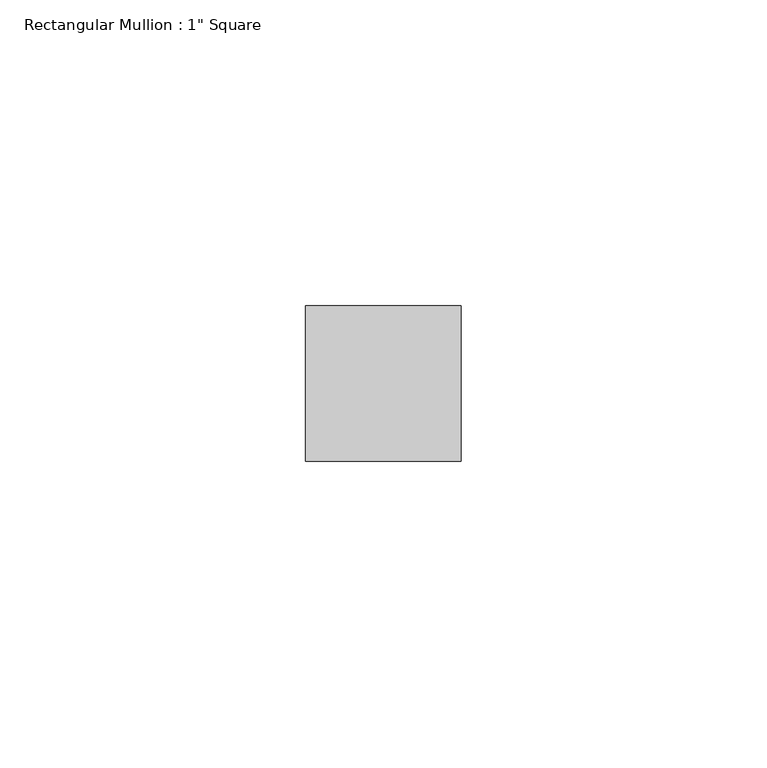
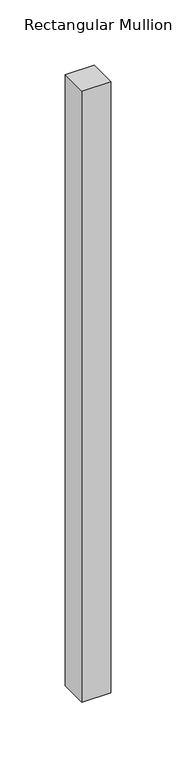
"""IFC4 building model written with IfcOpenShell, lengths in millimetres: member geometry."""

from ifc_helpers import new_model, si_unit, frame, origin, place, context, project, spatial, polyline, outline, extrude, source, transform, mapped, element, save


def member_030db1c4(model_context):
    return source(origin(), model_context, "Body", "SweptSolid", [
        extrude(outline(polyline([(0.0, 12.7), (0.0, -12.7), (-25.4, -12.7), (-25.4, 12.7), (0.0, 12.7)])), frame((0.0, 0.0, -571.5), z_axis=(0.0, 0.0, 1.0), x_axis=(1.0, 0.0, 0.0)), (0.0, 0.0, 1.0), 571.5),
    ])


if __name__ == "__main__":
    model = new_model("IFC4")
    model_context = context("Model", 3, world=origin())
    ifc_project = project(units=[si_unit("LENGTHUNIT", "METRE", prefix="MILLI")], contexts=[model_context])
    site = spatial("IfcSite", under=ifc_project)
    building = spatial("IfcBuilding", under=site)
    placement = place(None, origin())
    member_shape = member_030db1c4(model_context)
    element("IfcMember", 1, ObjectType="Rectangular Mullion : 1\" Square", at=placement, inside=building, context=model_context, shape_type="MappedRepresentation", body=[
        mapped(member_shape, transform((0.0, 0.0, 0.0), x_axis=(1.0, 0.0, 0.0), y_axis=(0.0, 1.0, 0.0), z_axis=(0.0, 0.0, 1.0))),
    ])
    save(model, "model.ifc")

# Revit data of these elements
# Type "Rectangular Mullion : 1\" Square"
#   built-in parameter 1007304 = 0.0833333 (stored number, unit not read)
#   built-in parameter 1007301 = 0.0416667 (stored number, unit not read)
#   built-in parameter 1007300 = 0.0416667 (stored number, unit not read)
# Element 1 (IfcMember, "Rectangular Mullion : 1\" Square")
#   Materials on its faces: "Metal - Aluminum"
# Materials
#   "Metal - Aluminum": class "Metal", colour RGB 247 247 247, transparency 0
